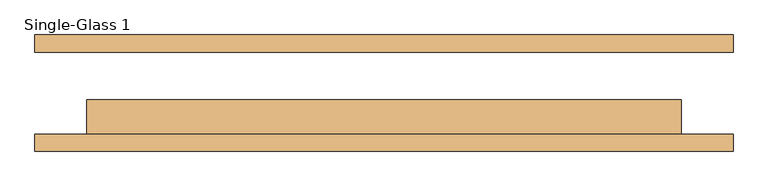
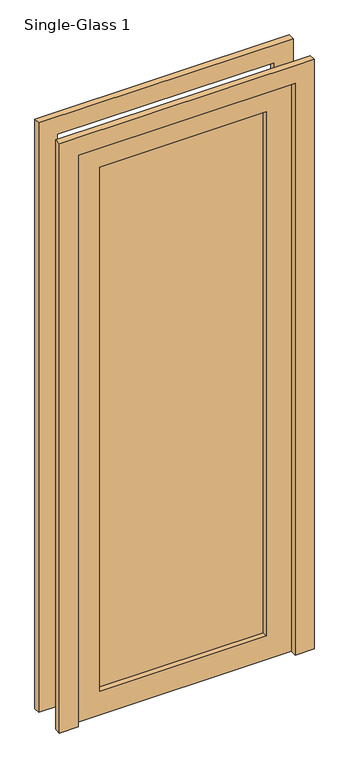
"""IFC4 building model written with IfcOpenShell, lengths in millimetres: door geometry, Single-Glass 1."""

from ifc_helpers import new_model, si_unit, frame, origin, place, context, project, spatial, polyline, outline, extrude, source, transform, mapped, element, save


def single_glass_1_90777ae4(model_context):
    return source(origin(), model_context, "Body", "SweptSolid", [
        extrude(outline(polyline([(2438.4, 437.35625), (0.0, 437.35625), (0.0, 513.55625), (2514.6, 513.55625), (2514.6, -513.55625), (0.0, -513.55625), (0.0, -437.35625), (2438.4, -437.35625), (2438.4, 437.35625)])), frame((0.0, 60.325, 0.0), z_axis=(0.0, 1.0, 0.0), x_axis=(0.0, 0.0, 1.0)), (0.0, 0.0, 1.0), 25.4),
        extrude(outline(polyline([(2438.4, 437.35625), (0.0, 437.35625), (0.0, 513.55625), (2514.6, 513.55625), (2514.6, -513.55625), (0.0, -513.55625), (0.0, -437.35625), (2438.4, -437.35625), (2438.4, 437.35625)])), frame((0.0, -85.725, 0.0), z_axis=(0.0, 1.0, 0.0), x_axis=(0.0, 0.0, 1.0)), (0.0, 0.0, 1.0), 25.4),
        extrude(outline(polyline([(335.75625, -31.75), (335.75625, -38.1), (-335.75625, -38.1), (-335.75625, -31.75), (335.75625, -31.75)])), frame((0.0, 0.0, 101.6), z_axis=(0.0, 0.0, 1.0), x_axis=(1.0, 0.0, 0.0)), (0.0, 0.0, 1.0), 2235.2),
        extrude(outline(polyline([(2438.4, 437.35625), (2438.4, -437.35625), (0.0, -437.35625), (0.0, 437.35625), (2438.4, 437.35625)]), holes=[polyline([(2336.8, -335.75625), (2336.8, 335.75625), (101.6, 335.75625), (101.6, -335.75625), (2336.8, -335.75625)])]), frame((0.0, -60.325, 0.0), z_axis=(0.0, 1.0, 0.0), x_axis=(0.0, 0.0, 1.0)), (0.0, 0.0, 1.0), 50.8),
    ])


if __name__ == "__main__":
    model = new_model("IFC4")
    model_context = context("Model", 3, world=origin())
    ifc_project = project(units=[si_unit("LENGTHUNIT", "METRE", prefix="MILLI")], contexts=[model_context])
    site = spatial("IfcSite", under=ifc_project)
    building = spatial("IfcBuilding", under=site)
    placement = place(None, origin())
    single_glass_1_shape = single_glass_1_90777ae4(model_context)
    element("IfcDoor", 1, ObjectType="Single-Glass 1 : 2'  10 7/16\" x96\"", at=placement, inside=building, context=model_context, shape_type="MappedRepresentation", body=[
        mapped(single_glass_1_shape, transform((0.0, 0.0, 0.0), x_axis=(1.0, 0.0, 0.0), y_axis=(0.0, 1.0, 0.0), z_axis=(0.0, 0.0, 1.0))),
    ])
    save(model, "model.ifc")

# Revit data of these elements
# Type "Single-Glass 1 : 2'  10 7/16\" x96\""
#   Type Mark = "41"
#   Construction Type Id = "MDOOR"
#   Assembly Code = "C1020"
#   Analytic Construction = "Metal"
#   Thickness = 0' - 2"
#   Heat Transfer Coefficient (U) = 3.7021 W/(m²·K)
#   Height = 8' - 0"
#   Rail Width - Base = 0' - 4"
#   Rail Width - Top = 0' - 4"
#   Stile Width - Hinge = 0' - 4"
#   Stile Width - Latch = 0' - 4"
#   Trim Projection Ext = 0' - 1"
#   Trim Projection Int = 0' - 1"
#   Trim Width = 0' - 3"
#   Width = 2' - 10 7/16"
#   Door Material = INTERIOR GRADE ALUMINUM STOREFRONT W/ SAFETY GLAZING
#   Frame Material = INTERIOR GRADE ALUMINUM STOREFRONT W/ SAFETY GLAZING
#   Visual Light Transmittance = 0
#   Solar Heat Gain Coefficient = 0
#   Function = (empty or 0)
#   Wall Closure = (empty or 0)
# Element 1 (IfcDoor, "Single-Glass 1 : 2'  10 7/16\" x96\"")
#   Materials on its faces: "INTERIOR GRADE ALUMINUM STOREFRONT W/ SAFETY GLAZING", "SAFETY GLAZING"
# Materials
#   "INTERIOR GRADE ALUMINUM STOREFRONT W/ SAFETY GLAZING": class "Metal", colour RGB 226 226 226, transparency 0, Description = "Aluminum 6061", Cost = 0
#   "SAFETY GLAZING": class "Glass", colour RGB 142 168 196, transparency 0.75, Description = "Soda Lime Glass", Cost = 0
